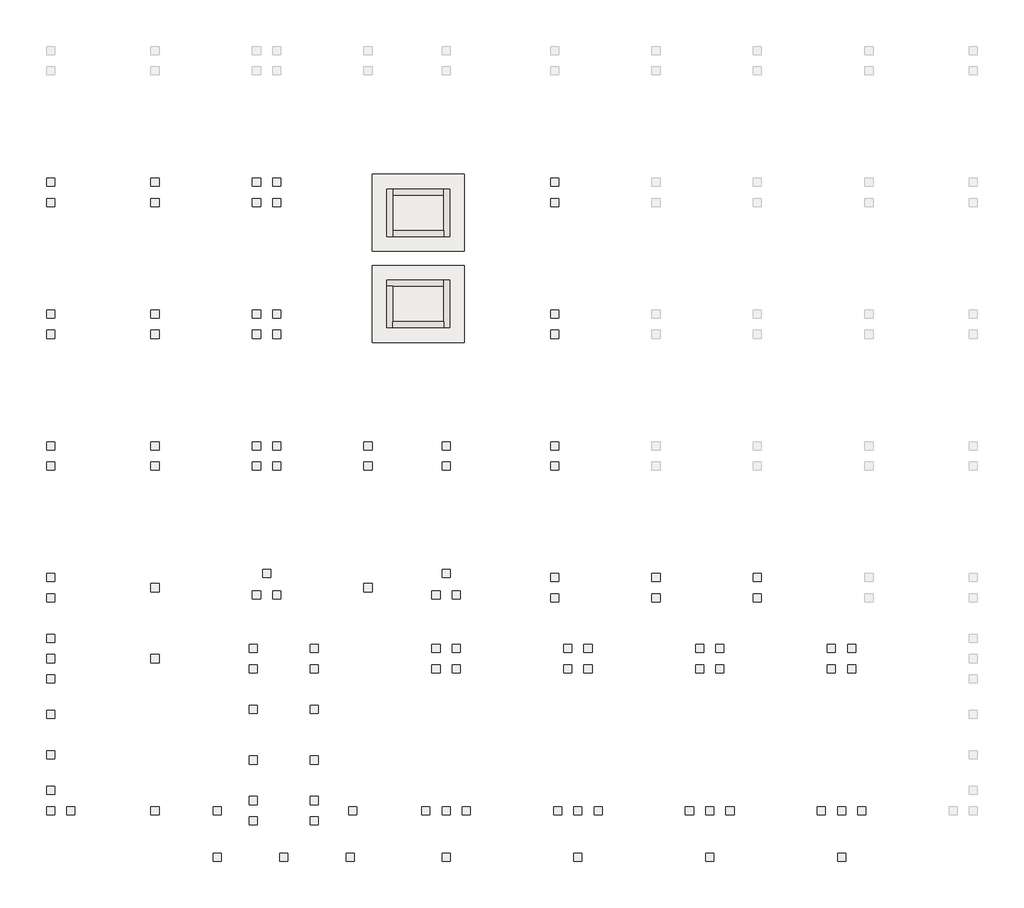
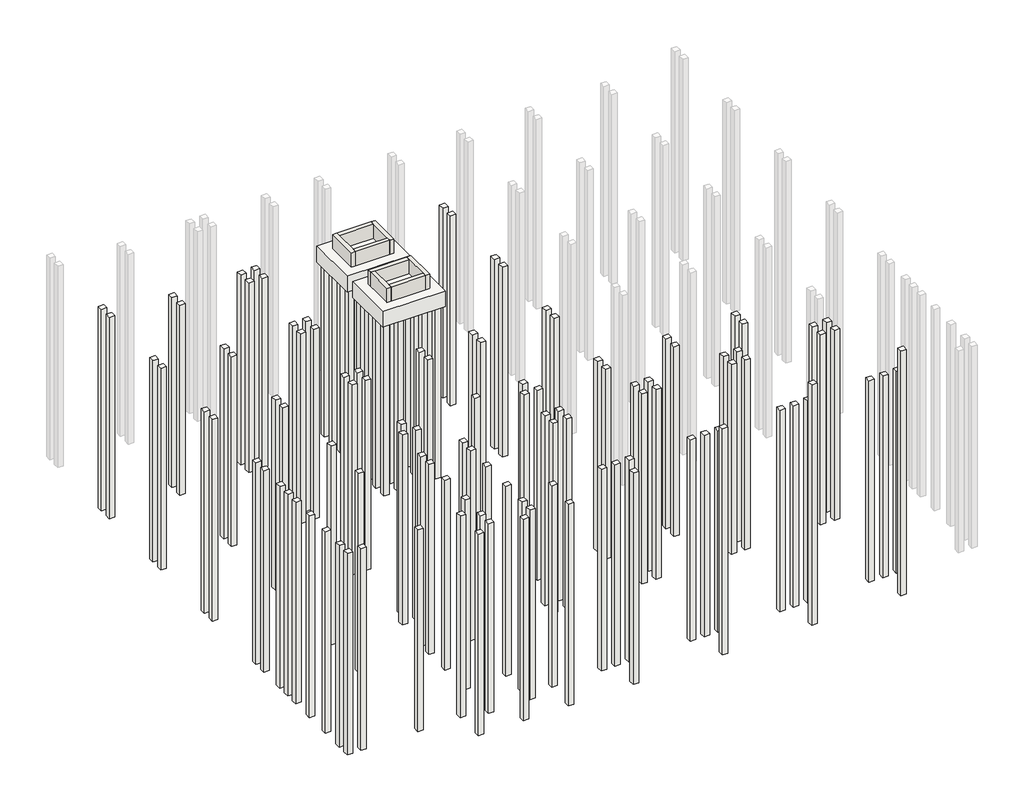
# Not in any storey, part 1 of 2: 143 slabs, 8 walls.
"""IFC4 building model written with IfcOpenShell, lengths in millimetres."""

import ifcopenshell
import ifcopenshell.guid

model = None  # the IFC model being written
_history = None  # IfcOwnerHistory: only IFC2X3 demands one
_inside = {}  # id of a spatial element -> (the spatial element, [elements in it])
_under = {}  # id of a project, library or spatial element -> (it, [spatial elements below it])
_declared = {}  # id of a project -> (the project, [libraries it declares])
_typed = {}  # id of a type object -> (the type object, [elements of that type])
_made_of = {}  # id of a material, layer set ... -> (it, [elements and type objects made of it])


def new_model(schema):
    """Start an empty IFC model of exactly this schema.

    Asked for "IFC4X3", IfcOpenShell would pick the latest addendum, in which some entities
    have other attributes; the version numbers below select the first issue.
    IFC2X3 requires an IfcOwnerHistory on every rooted entity: one is made here for all.
    """
    global model, _history
    if schema == "IFC4X3":
        model = ifcopenshell.file(schema_version=(4, 3, 0, 0))
    else:
        model = ifcopenshell.file(schema=schema)
    _inside.clear()
    _under.clear()
    _declared.clear()
    _typed.clear()
    _made_of.clear()
    _history = None
    if model.schema == "IFC2X3":
        org = make("IfcOrganization", Name="unknown")
        user = make(
            "IfcPersonAndOrganization",
            ThePerson=make("IfcPerson", FamilyName="unknown"),
            TheOrganization=org,
        )
        app = make(
            "IfcApplication",
            ApplicationDeveloper=org,
            Version="unknown",
            ApplicationFullName="unknown",
            ApplicationIdentifier="unknown",
        )
        _history = make(
            "IfcOwnerHistory",
            OwningUser=user,
            OwningApplication=app,
            ChangeAction="ADDED",
            CreationDate=0,
        )
    return model


def make(cls, **values):
    """One entity of the class cls with the attributes given. An attribute that is None is left unset."""
    return model.create_entity(
        cls, **{name: value for name, value in values.items() if value is not None}
    )


def rooted(cls, **values):
    """An entity with a GlobalId (a new one), such as an element, a storey or a relation."""
    return make(cls, GlobalId=ifcopenshell.guid.new(), OwnerHistory=_history, **values)


def si_unit(unit_type, name, prefix=None):
    """IfcSIUnit, for example si_unit("LENGTHUNIT", "METRE", prefix="MILLI")."""
    return make("IfcSIUnit", UnitType=unit_type, Prefix=prefix, Name=name)


def assignment(units):
    """IfcUnitAssignment: the units of a project."""
    return None if units is None else make("IfcUnitAssignment", Units=units)


def point(xyz):
    """IfcCartesianPoint."""
    return None if xyz is None else make("IfcCartesianPoint", Coordinates=xyz)


def direction(xyz):
    """IfcDirection."""
    return None if xyz is None else make("IfcDirection", DirectionRatios=xyz)


def frame(location, z_axis=None, x_axis=None):
    """IfcAxis2Placement3D, a coordinate frame: its origin and axes. An axis left out is left unset."""
    return make(
        "IfcAxis2Placement3D",
        Location=point(location),
        Axis=direction(z_axis),
        RefDirection=direction(x_axis),
    )


def origin():
    """The frame at (0, 0, 0) with its axes left unset."""
    return frame((0.0, 0.0, 0.0))


def place(relative_to, where):
    """IfcLocalPlacement: puts the frame where relative to a parent placement (None: the world)."""
    return make(
        "IfcLocalPlacement", PlacementRelTo=relative_to, RelativePlacement=where
    )


def context(
    kind, dimensions, precision=None, world=None, true_north=None, identifier=None
):
    """IfcGeometricRepresentationContext, for example the 3D "Model" context."""
    return make(
        "IfcGeometricRepresentationContext",
        ContextIdentifier=identifier,
        ContextType=kind,
        CoordinateSpaceDimension=dimensions,
        Precision=precision,
        WorldCoordinateSystem=world,
        TrueNorth=true_north,
    )


def project(units=None, contexts=None):
    """IfcProject with its units and contexts."""
    return rooted(
        "IfcProject",
        Name="project",
        RepresentationContexts=contexts,
        UnitsInContext=assignment(units),
    )


def spatial(cls, under=None, at=None, **own):
    """A site, building, storey or space (cls), placed at a placement, below another one or the project."""
    s = rooted(cls, ObjectPlacement=at, **own)
    if under is not None:
        _under.setdefault(under.id(), (under, []))[1].append(s)
    return s


def polyline(points):
    """IfcPolyline through the points."""
    return make("IfcPolyline", Points=[point(p) for p in points])


def outline(outer, holes=None, kind="AREA"):
    """IfcArbitraryClosedProfileDef: a profile drawn as a closed curve; with holes, ...WithVoids."""
    if holes is None:
        return make("IfcArbitraryClosedProfileDef", ProfileType=kind, OuterCurve=outer)
    return make(
        "IfcArbitraryProfileDefWithVoids",
        ProfileType=kind,
        OuterCurve=outer,
        InnerCurves=holes,
    )


def extrude(swept, where, along, depth):
    """IfcExtrudedAreaSolid: the profile swept, set in the frame where, extruded along a direction by depth."""
    return make(
        "IfcExtrudedAreaSolid",
        SweptArea=swept,
        Position=where,
        ExtrudedDirection=direction(along),
        Depth=depth,
    )


def faces_of(points, faces, orient=None, outer=None):
    """IfcFace entities. A face is a list of loops; a loop is a list of indices into points, from 0.

    orient and outer hold one flag for each loop. By default every Orientation is true, the
    first loop of a face is its IfcFaceOuterBound and the others are IfcFaceBound.
    """
    made = []
    for i, loops in enumerate(faces):
        bounds = []
        for j, loop in enumerate(loops):
            is_outer = j == 0 if outer is None else outer[i][j]
            bounds.append(
                make(
                    "IfcFaceOuterBound" if is_outer else "IfcFaceBound",
                    Bound=make("IfcPolyLoop", Polygon=[points[k] for k in loop]),
                    Orientation=True if orient is None else orient[i][j],
                )
            )
        made.append(make("IfcFace", Bounds=bounds))
    return made


def faceted_brep(points, faces, orient=None, outer=None, voids=None):
    """IfcFacetedBrep: a solid bounded by flat faces; with voids (closed shells), ...WithVoids."""
    shared = [point(p) for p in points]
    hull = make("IfcClosedShell", CfsFaces=faces_of(shared, faces, orient, outer))
    if voids is None:
        return make("IfcFacetedBrep", Outer=hull)
    return make(
        "IfcFacetedBrepWithVoids",
        Outer=hull,
        Voids=[
            make(cls, CfsFaces=faces_of(shared, fs, o, b)) for cls, fs, o, b in voids
        ],
    )


def shape(context_of_items, identifier, shape_type, items):
    """IfcShapeRepresentation: the items that make up one representation, for example the "Body"."""
    return make(
        "IfcShapeRepresentation",
        ContextOfItems=context_of_items,
        RepresentationIdentifier=identifier,
        RepresentationType=shape_type,
        Items=items,
    )


def source(mapping_origin, context_of_items, identifier, shape_type, items):
    """IfcRepresentationMap: a shape defined once, which mapped items show again and again."""
    return make(
        "IfcRepresentationMap",
        MappingOrigin=mapping_origin,
        MappedRepresentation=shape(context_of_items, identifier, shape_type, items),
    )


def transform(
    local_origin,
    x_axis=None,
    y_axis=None,
    z_axis=None,
    scale=None,
    scale2=None,
    scale3=None,
    uniform=True,
):
    """IfcCartesianTransformationOperator3D, or its non-uniform kind. x_axis, y_axis, z_axis: its Axis1, 2, 3."""
    if uniform:
        return make(
            "IfcCartesianTransformationOperator3D",
            Axis1=direction(x_axis),
            Axis2=direction(y_axis),
            LocalOrigin=point(local_origin),
            Scale=scale,
            Axis3=direction(z_axis),
        )
    return make(
        "IfcCartesianTransformationOperator3DnonUniform",
        Axis1=direction(x_axis),
        Axis2=direction(y_axis),
        LocalOrigin=point(local_origin),
        Scale=scale,
        Axis3=direction(z_axis),
        Scale2=scale2,
        Scale3=scale3,
    )


def mapped(mapping_source, mapping_target):
    """IfcMappedItem: shows the shape of a source again, moved by a transform."""
    return make(
        "IfcMappedItem", MappingSource=mapping_source, MappingTarget=mapping_target
    )


def made_of(thing, what):
    """Note that an element or type object is made of a material, layer set ...; save() writes the relation."""
    if what is not None:
        _made_of.setdefault(what.id(), (what, []))[1].append(thing)
    return thing


def element(
    cls,
    number,
    at=None,
    inside=None,
    cuts=None,
    type_object=None,
    material=None,
    context=None,
    identifier="Body",
    shape_type=None,
    held_by="IfcProductDefinitionShape",
    body=None,
    shapes=None,
    **own,
):
    """One element of the class cls, such as IfcWall. Its Tag is "e" and its number.

    at: its placement. inside: the storey or other place that contains it. cuts: it is an
    opening in that element (IfcRelVoidsElement). A single representation is given by context,
    identifier, shape_type and body (its items); several are given by shapes. held_by: the class
    of the entity that holds the representations. save() writes the other relations.
    """
    e = rooted(cls, Tag="e%d" % number, ObjectPlacement=at, **own)
    if body is not None:
        shapes = [shape(context, identifier, shape_type, body)]
    if shapes is not None:
        e.Representation = make(held_by, Representations=shapes)
    if inside is not None:
        _inside.setdefault(inside.id(), (inside, []))[1].append(e)
    if cuts is not None:
        rooted(
            "IfcRelVoidsElement", RelatingBuildingElement=cuts, RelatedOpeningElement=e
        )
    if type_object is not None:
        _typed.setdefault(type_object.id(), (type_object, []))[1].append(e)
    return made_of(e, material)


def aggregate(whole, parts):
    """IfcRelAggregates: a whole, such as a stair, and the parts it consists of."""
    return rooted("IfcRelAggregates", RelatingObject=whole, RelatedObjects=parts)


def save(model, path):
    """Write the relations noted so far, then the file.

    IfcRelAggregates (storeys below a building ...), IfcRelContainedInSpatialStructure (elements
    in a storey), IfcRelDefinesByType, IfcRelAssociatesMaterial and IfcRelDeclares: one each for
    every whole, place, type object, material and project.
    """
    for whole, parts in _under.values():
        aggregate(whole, parts)
    for where, things in _inside.values():
        rooted(
            "IfcRelContainedInSpatialStructure",
            RelatedElements=things,
            RelatingStructure=where,
        )
    for kind, things in _typed.values():
        rooted("IfcRelDefinesByType", RelatedObjects=things, RelatingType=kind)
    for what, things in _made_of.values():
        rooted("IfcRelAssociatesMaterial", RelatedObjects=things, RelatingMaterial=what)
    for by, libraries in _declared.values():
        rooted("IfcRelDeclares", RelatingContext=by, RelatedDefinitions=libraries)
    model.write(path)


def slab_e3f33549(model_context):
    return source(origin(), model_context, "Body", "SweptSolid", [
        extrude(outline(polyline([(200.0, -200.0), (-200.0, -200.0), (-200.0, 200.0), (200.0, 200.0), (200.0, -200.0)])), frame((0.0, 0.0, -20000.0), z_axis=(0.0, 0.0, 1.0), x_axis=(1.0, 0.0, 0.0)), (0.0, 0.0, 1.0), 15320.0),
    ])


def slab_2462c6b3(model_context):
    return source(origin(), model_context, "Body", "SweptSolid", [
        extrude(outline(polyline([(200.0, -200.0), (-200.0, -200.0), (-200.0, 200.0), (200.0, 200.0), (200.0, -200.0)])), frame((0.0, 0.0, -20000.0), z_axis=(0.0, 0.0, 1.0), x_axis=(1.0, 0.0, 0.0)), (0.0, 0.0, 1.0), 14620.0),
    ])


def slab_4eaa82be(model_context):
    return source(origin(), model_context, "Body", "SweptSolid", [
        extrude(outline(polyline([(200.0, -200.0), (-200.0, -200.0), (-200.0, 200.0), (200.0, 200.0), (200.0, -200.0)])), frame((0.0, 0.0, -20000.0), z_axis=(0.0, 0.0, 1.0), x_axis=(1.0, 0.0, 0.0)), (0.0, 0.0, 1.0), 15520.0),
    ])


def slab_98706cf3(model_context):
    return source(origin(), model_context, "Body", "SweptSolid", [
        extrude(outline(polyline([(200.0, -200.0), (-200.0, -200.0), (-200.0, 200.0), (200.0, 200.0), (200.0, -200.0)])), frame((0.0, 0.0, -20000.0), z_axis=(0.0, 0.0, 1.0), x_axis=(1.0, 0.0, 0.0)), (0.0, 0.0, 1.0), 16280.0),
    ])


def slab_73a1868d(model_context):
    return source(origin(), model_context, "Body", "SweptSolid", [
        extrude(outline(polyline([(200.0, -200.0), (-200.0, -200.0), (-200.0, 200.0), (200.0, 200.0), (200.0, -200.0)])), frame((0.0, 0.0, -20000.0), z_axis=(0.0, 0.0, 1.0), x_axis=(1.0, 0.0, 0.0)), (0.0, 0.0, 1.0), 17400.0),
    ])


def slab_81e4ded3(model_context):
    return source(origin(), model_context, "Body", "SweptSolid", [
        extrude(outline(polyline([(200.0, -200.0), (-200.0, -200.0), (-200.0, 200.0), (200.0, 200.0), (200.0, -200.0)])), frame((0.0, 0.0, -20000.0), z_axis=(0.0, 0.0, 1.0), x_axis=(1.0, 0.0, 0.0)), (0.0, 0.0, 1.0), 18520.0),
    ])


def slab_0d914d5e(model_context):
    return source(origin(), model_context, "Body", "SweptSolid", [
        extrude(outline(polyline([(200.0, -200.0), (-200.0, -200.0), (-200.0, 200.0), (200.0, 200.0), (200.0, -200.0)])), frame((0.0, 0.0, -20000.0), z_axis=(0.0, 0.0, 1.0), x_axis=(1.0, 0.0, 0.0)), (0.0, 0.0, 1.0), 18850.0),
    ])


def slab_443494b9(model_context):
    return source(origin(), model_context, "Body", "SweptSolid", [
        extrude(outline(polyline([(200.0, -200.0), (-200.0, -200.0), (-200.0, 200.0), (200.0, 200.0), (200.0, -200.0)])), frame((0.0, 0.0, -20000.0), z_axis=(0.0, 0.0, 1.0), x_axis=(1.0, 0.0, 0.0)), (0.0, 0.0, 1.0), 13220.0),
    ])


model = new_model("IFC4")

# Units and contexts
model_context = context("Model", 3, world=origin())
ifc_project = project(units=[si_unit("LENGTHUNIT", "METRE", prefix="MILLI")], contexts=[model_context])

# Site, building
site = spatial("IfcSite", under=ifc_project)
building = spatial("IfcBuilding", under=site)

# Slabs
placement = place(None, origin())
element("IfcSlab", 1, at=placement, inside=building, context=model_context, shape_type="SweptSolid", body=[
    extrude(outline(polyline([(22350.0, 27600.0), (22350.0, 31400.0), (26900.0, 31400.0), (26900.0, 27600.0), (22350.0, 27600.0)])), frame((0.0, 0.0, -6800.0), z_axis=(0.0, 0.0, 1.0), x_axis=(1.0, 0.0, 0.0)), (0.0, 0.0, 1.0), 1200.0),
])
element("IfcSlab", 2, at=placement, inside=building, context=model_context, shape_type="SweptSolid", body=[
    extrude(outline(polyline([(22350.0, 23100.0), (22350.0, 26900.0), (26900.0, 26900.0), (26900.0, 23100.0), (22350.0, 23100.0)])), frame((0.0, 0.0, -6800.0), z_axis=(0.0, 0.0, 1.0), x_axis=(1.0, 0.0, 0.0)), (0.0, 0.0, 1.0), 1200.0),
])
slab_shape = slab_e3f33549(model_context)
element("IfcSlab", 3, at=placement, inside=building, context=model_context, shape_type="MappedRepresentation", body=[
    mapped(slab_shape, transform((11650.0, 7500.0, 0.0), x_axis=(1.0, 0.0, 0.0), y_axis=(0.0, 1.0, 0.0), z_axis=(0.0, 0.0, 1.0))),
])
element("IfcSlab", 4, at=placement, inside=building, context=model_context, shape_type="MappedRepresentation", body=[
    mapped(slab_shape, transform((11650.0, 11000.0, 0.0), x_axis=(1.0, 0.0, 0.0), y_axis=(0.0, 1.0, 0.0), z_axis=(0.0, 0.0, 1.0))),
])
element("IfcSlab", 5, at=placement, inside=building, context=model_context, shape_type="MappedRepresentation", body=[
    mapped(slab_shape, transform((22150.0, 11000.0, 0.0), x_axis=(1.0, 0.0, 0.0), y_axis=(0.0, 1.0, 0.0), z_axis=(0.0, 0.0, 1.0))),
])
slab_2_shape = slab_2462c6b3(model_context)
element("IfcSlab", 6, at=placement, inside=building, context=model_context, shape_type="MappedRepresentation", body=[
    mapped(slab_2_shape, transform((22150.0, 17000.0, 0.0), x_axis=(1.0, 0.0, 0.0), y_axis=(0.0, 1.0, 0.0), z_axis=(0.0, 0.0, 1.0))),
])
element("IfcSlab", 7, at=placement, inside=building, context=model_context, shape_type="MappedRepresentation", body=[
    mapped(slab_2_shape, transform((22150.0, 18000.0, 0.0), x_axis=(1.0, 0.0, 0.0), y_axis=(0.0, 1.0, 0.0), z_axis=(0.0, 0.0, 1.0))),
])
element("IfcSlab", 8, at=placement, inside=building, context=model_context, shape_type="MappedRepresentation", body=[
    mapped(slab_2_shape, transform((26000.0, 17000.0, 0.0), x_axis=(1.0, 0.0, 0.0), y_axis=(0.0, 1.0, 0.0), z_axis=(0.0, 0.0, 1.0))),
])
element("IfcSlab", 9, at=placement, inside=building, context=model_context, shape_type="MappedRepresentation", body=[
    mapped(slab_2_shape, transform((26000.0, 18000.0, 0.0), x_axis=(1.0, 0.0, 0.0), y_axis=(0.0, 1.0, 0.0), z_axis=(0.0, 0.0, 1.0))),
])
element("IfcSlab", 10, at=placement, inside=building, context=model_context, shape_type="MappedRepresentation", body=[
    mapped(slab_2_shape, transform((11650.0, 17000.0, 0.0), x_axis=(1.0, 0.0, 0.0), y_axis=(0.0, 1.0, 0.0), z_axis=(0.0, 0.0, 1.0))),
])
element("IfcSlab", 11, at=placement, inside=building, context=model_context, shape_type="MappedRepresentation", body=[
    mapped(slab_2_shape, transform((11650.0, 18000.0, 0.0), x_axis=(1.0, 0.0, 0.0), y_axis=(0.0, 1.0, 0.0), z_axis=(0.0, 0.0, 1.0))),
])
element("IfcSlab", 12, at=placement, inside=building, context=model_context, shape_type="MappedRepresentation", body=[
    mapped(slab_2_shape, transform((11650.0, 23500.0, 0.0), x_axis=(1.0, 0.0, 0.0), y_axis=(0.0, 1.0, 0.0), z_axis=(0.0, 0.0, 1.0))),
])
element("IfcSlab", 13, at=placement, inside=building, context=model_context, shape_type="MappedRepresentation", body=[
    mapped(slab_2_shape, transform((11650.0, 24500.0, 0.0), x_axis=(1.0, 0.0, 0.0), y_axis=(0.0, 1.0, 0.0), z_axis=(0.0, 0.0, 1.0))),
])
element("IfcSlab", 14, at=placement, inside=building, context=model_context, shape_type="MappedRepresentation", body=[
    mapped(slab_2_shape, transform((11650.0, 30000.0, 0.0), x_axis=(1.0, 0.0, 0.0), y_axis=(0.0, 1.0, 0.0), z_axis=(0.0, 0.0, 1.0))),
])
element("IfcSlab", 15, at=placement, inside=building, context=model_context, shape_type="MappedRepresentation", body=[
    mapped(slab_2_shape, transform((11650.0, 31000.0, 0.0), x_axis=(1.0, 0.0, 0.0), y_axis=(0.0, 1.0, 0.0), z_axis=(0.0, 0.0, 1.0))),
])
element("IfcSlab", 16, at=placement, inside=building, context=model_context, shape_type="MappedRepresentation", body=[
    mapped(slab_2_shape, transform((31350.0, 10500.0, 0.0), x_axis=(1.0, 0.0, 0.0), y_axis=(0.0, 1.0, 0.0), z_axis=(0.0, 0.0, 1.0))),
])
element("IfcSlab", 17, at=placement, inside=building, context=model_context, shape_type="MappedRepresentation", body=[
    mapped(slab_2_shape, transform((31350.0, 11500.0, 0.0), x_axis=(1.0, 0.0, 0.0), y_axis=(0.0, 1.0, 0.0), z_axis=(0.0, 0.0, 1.0))),
])
element("IfcSlab", 18, at=placement, inside=building, context=model_context, shape_type="MappedRepresentation", body=[
    mapped(slab_2_shape, transform((36350.0, 10500.0, 0.0), x_axis=(1.0, 0.0, 0.0), y_axis=(0.0, 1.0, 0.0), z_axis=(0.0, 0.0, 1.0))),
])
element("IfcSlab", 19, at=placement, inside=building, context=model_context, shape_type="MappedRepresentation", body=[
    mapped(slab_2_shape, transform((36350.0, 11500.0, 0.0), x_axis=(1.0, 0.0, 0.0), y_axis=(0.0, 1.0, 0.0), z_axis=(0.0, 0.0, 1.0))),
])
element("IfcSlab", 20, at=placement, inside=building, context=model_context, shape_type="MappedRepresentation", body=[
    mapped(slab_2_shape, transform((41350.0, 10500.0, 0.0), x_axis=(1.0, 0.0, 0.0), y_axis=(0.0, 1.0, 0.0), z_axis=(0.0, 0.0, 1.0))),
])
element("IfcSlab", 21, at=placement, inside=building, context=model_context, shape_type="MappedRepresentation", body=[
    mapped(slab_2_shape, transform((41350.0, 11500.0, 0.0), x_axis=(1.0, 0.0, 0.0), y_axis=(0.0, 1.0, 0.0), z_axis=(0.0, 0.0, 1.0))),
])
element("IfcSlab", 22, at=placement, inside=building, context=model_context, shape_type="MappedRepresentation", body=[
    mapped(slab_2_shape, transform((46000.0, 7000.0, 0.0), x_axis=(1.0, 0.0, 0.0), y_axis=(0.0, 1.0, 0.0), z_axis=(0.0, 0.0, 1.0))),
])
element("IfcSlab", 23, at=placement, inside=building, context=model_context, shape_type="MappedRepresentation", body=[
    mapped(slab_2_shape, transform((46000.0, 8000.0, 0.0), x_axis=(1.0, 0.0, 0.0), y_axis=(0.0, 1.0, 0.0), z_axis=(0.0, 0.0, 1.0))),
])
element("IfcSlab", 24, at=placement, inside=building, context=model_context, shape_type="MappedRepresentation", body=[
    mapped(slab_2_shape, transform((45000.0, 7000.0, 0.0), x_axis=(1.0, 0.0, 0.0), y_axis=(0.0, 1.0, 0.0), z_axis=(0.0, 0.0, 1.0))),
])
element("IfcSlab", 25, at=placement, inside=building, context=model_context, shape_type="MappedRepresentation", body=[
    mapped(slab_2_shape, transform((45000.0, 8000.0, 0.0), x_axis=(1.0, 0.0, 0.0), y_axis=(0.0, 1.0, 0.0), z_axis=(0.0, 0.0, 1.0))),
])
element("IfcSlab", 26, at=placement, inside=building, context=model_context, shape_type="MappedRepresentation", body=[
    mapped(slab_2_shape, transform((39500.0, 7000.0, 0.0), x_axis=(1.0, 0.0, 0.0), y_axis=(0.0, 1.0, 0.0), z_axis=(0.0, 0.0, 1.0))),
])
element("IfcSlab", 27, at=placement, inside=building, context=model_context, shape_type="MappedRepresentation", body=[
    mapped(slab_2_shape, transform((39500.0, 8000.0, 0.0), x_axis=(1.0, 0.0, 0.0), y_axis=(0.0, 1.0, 0.0), z_axis=(0.0, 0.0, 1.0))),
])
element("IfcSlab", 28, at=placement, inside=building, context=model_context, shape_type="MappedRepresentation", body=[
    mapped(slab_2_shape, transform((38500.0, 7000.0, 0.0), x_axis=(1.0, 0.0, 0.0), y_axis=(0.0, 1.0, 0.0), z_axis=(0.0, 0.0, 1.0))),
])
element("IfcSlab", 29, at=placement, inside=building, context=model_context, shape_type="MappedRepresentation", body=[
    mapped(slab_2_shape, transform((38500.0, 8000.0, 0.0), x_axis=(1.0, 0.0, 0.0), y_axis=(0.0, 1.0, 0.0), z_axis=(0.0, 0.0, 1.0))),
])
element("IfcSlab", 30, at=placement, inside=building, context=model_context, shape_type="MappedRepresentation", body=[
    mapped(slab_2_shape, transform((33000.0, 7000.0, 0.0), x_axis=(1.0, 0.0, 0.0), y_axis=(0.0, 1.0, 0.0), z_axis=(0.0, 0.0, 1.0))),
])
element("IfcSlab", 31, at=placement, inside=building, context=model_context, shape_type="MappedRepresentation", body=[
    mapped(slab_2_shape, transform((33000.0, 8000.0, 0.0), x_axis=(1.0, 0.0, 0.0), y_axis=(0.0, 1.0, 0.0), z_axis=(0.0, 0.0, 1.0))),
])
element("IfcSlab", 32, at=placement, inside=building, context=model_context, shape_type="MappedRepresentation", body=[
    mapped(slab_2_shape, transform((32000.0, 7000.0, 0.0), x_axis=(1.0, 0.0, 0.0), y_axis=(0.0, 1.0, 0.0), z_axis=(0.0, 0.0, 1.0))),
])
element("IfcSlab", 33, at=placement, inside=building, context=model_context, shape_type="MappedRepresentation", body=[
    mapped(slab_2_shape, transform((32000.0, 8000.0, 0.0), x_axis=(1.0, 0.0, 0.0), y_axis=(0.0, 1.0, 0.0), z_axis=(0.0, 0.0, 1.0))),
])
element("IfcSlab", 34, at=placement, inside=building, context=model_context, shape_type="MappedRepresentation", body=[
    mapped(slab_2_shape, transform((26500.0, 7000.0, 0.0), x_axis=(1.0, 0.0, 0.0), y_axis=(0.0, 1.0, 0.0), z_axis=(0.0, 0.0, 1.0))),
])
element("IfcSlab", 35, at=placement, inside=building, context=model_context, shape_type="MappedRepresentation", body=[
    mapped(slab_2_shape, transform((26500.0, 8000.0, 0.0), x_axis=(1.0, 0.0, 0.0), y_axis=(0.0, 1.0, 0.0), z_axis=(0.0, 0.0, 1.0))),
])
element("IfcSlab", 36, at=placement, inside=building, context=model_context, shape_type="MappedRepresentation", body=[
    mapped(slab_2_shape, transform((25500.0, 7000.0, 0.0), x_axis=(1.0, 0.0, 0.0), y_axis=(0.0, 1.0, 0.0), z_axis=(0.0, 0.0, 1.0))),
])
element("IfcSlab", 37, at=placement, inside=building, context=model_context, shape_type="MappedRepresentation", body=[
    mapped(slab_2_shape, transform((25500.0, 8000.0, 0.0), x_axis=(1.0, 0.0, 0.0), y_axis=(0.0, 1.0, 0.0), z_axis=(0.0, 0.0, 1.0))),
])
element("IfcSlab", 38, at=placement, inside=building, context=model_context, shape_type="MappedRepresentation", body=[
    mapped(slab_2_shape, transform((17650.0, 30000.0, 0.0), x_axis=(1.0, 0.0, 0.0), y_axis=(0.0, 1.0, 0.0), z_axis=(0.0, 0.0, 1.0))),
])
element("IfcSlab", 39, at=placement, inside=building, context=model_context, shape_type="MappedRepresentation", body=[
    mapped(slab_2_shape, transform((17650.0, 31000.0, 0.0), x_axis=(1.0, 0.0, 0.0), y_axis=(0.0, 1.0, 0.0), z_axis=(0.0, 0.0, 1.0))),
])
element("IfcSlab", 40, at=placement, inside=building, context=model_context, shape_type="MappedRepresentation", body=[
    mapped(slab_2_shape, transform((16650.0, 30000.0, 0.0), x_axis=(1.0, 0.0, 0.0), y_axis=(0.0, 1.0, 0.0), z_axis=(0.0, 0.0, 1.0))),
])
element("IfcSlab", 41, at=placement, inside=building, context=model_context, shape_type="MappedRepresentation", body=[
    mapped(slab_2_shape, transform((16650.0, 31000.0, 0.0), x_axis=(1.0, 0.0, 0.0), y_axis=(0.0, 1.0, 0.0), z_axis=(0.0, 0.0, 1.0))),
])
element("IfcSlab", 42, at=placement, inside=building, context=model_context, shape_type="MappedRepresentation", body=[
    mapped(slab_2_shape, transform((17650.0, 23500.0, 0.0), x_axis=(1.0, 0.0, 0.0), y_axis=(0.0, 1.0, 0.0), z_axis=(0.0, 0.0, 1.0))),
])
element("IfcSlab", 43, at=placement, inside=building, context=model_context, shape_type="MappedRepresentation", body=[
    mapped(slab_2_shape, transform((17650.0, 24500.0, 0.0), x_axis=(1.0, 0.0, 0.0), y_axis=(0.0, 1.0, 0.0), z_axis=(0.0, 0.0, 1.0))),
])
element("IfcSlab", 44, at=placement, inside=building, context=model_context, shape_type="MappedRepresentation", body=[
    mapped(slab_2_shape, transform((16650.0, 23500.0, 0.0), x_axis=(1.0, 0.0, 0.0), y_axis=(0.0, 1.0, 0.0), z_axis=(0.0, 0.0, 1.0))),
])
element("IfcSlab", 45, at=placement, inside=building, context=model_context, shape_type="MappedRepresentation", body=[
    mapped(slab_2_shape, transform((16650.0, 24500.0, 0.0), x_axis=(1.0, 0.0, 0.0), y_axis=(0.0, 1.0, 0.0), z_axis=(0.0, 0.0, 1.0))),
])
element("IfcSlab", 46, at=placement, inside=building, context=model_context, shape_type="MappedRepresentation", body=[
    mapped(slab_2_shape, transform((17650.0, 17000.0, 0.0), x_axis=(1.0, 0.0, 0.0), y_axis=(0.0, 1.0, 0.0), z_axis=(0.0, 0.0, 1.0))),
])
element("IfcSlab", 47, at=placement, inside=building, context=model_context, shape_type="MappedRepresentation", body=[
    mapped(slab_2_shape, transform((17650.0, 18000.0, 0.0), x_axis=(1.0, 0.0, 0.0), y_axis=(0.0, 1.0, 0.0), z_axis=(0.0, 0.0, 1.0))),
])
element("IfcSlab", 48, at=placement, inside=building, context=model_context, shape_type="MappedRepresentation", body=[
    mapped(slab_2_shape, transform((16650.0, 17000.0, 0.0), x_axis=(1.0, 0.0, 0.0), y_axis=(0.0, 1.0, 0.0), z_axis=(0.0, 0.0, 1.0))),
])
element("IfcSlab", 49, at=placement, inside=building, context=model_context, shape_type="MappedRepresentation", body=[
    mapped(slab_2_shape, transform((16650.0, 18000.0, 0.0), x_axis=(1.0, 0.0, 0.0), y_axis=(0.0, 1.0, 0.0), z_axis=(0.0, 0.0, 1.0))),
])
element("IfcSlab", 50, at=placement, inside=building, context=model_context, shape_type="MappedRepresentation", body=[
    mapped(slab_2_shape, transform((16650.0, 10650.0, 0.0), x_axis=(1.0, 0.0, 0.0), y_axis=(0.0, 1.0, 0.0), z_axis=(0.0, 0.0, 1.0))),
])
element("IfcSlab", 51, at=placement, inside=building, context=model_context, shape_type="MappedRepresentation", body=[
    mapped(slab_2_shape, transform((17650.0, 10650.0, 0.0), x_axis=(1.0, 0.0, 0.0), y_axis=(0.0, 1.0, 0.0), z_axis=(0.0, 0.0, 1.0))),
])
element("IfcSlab", 52, at=placement, inside=building, context=model_context, shape_type="MappedRepresentation", body=[
    mapped(slab_2_shape, transform((17150.0, 11700.0, 0.0), x_axis=(1.0, 0.0, 0.0), y_axis=(0.0, 1.0, 0.0), z_axis=(0.0, 0.0, 1.0))),
])
element("IfcSlab", 53, at=placement, inside=building, context=model_context, shape_type="MappedRepresentation", body=[
    mapped(slab_2_shape, transform((19500.0, 7000.0, 0.0), x_axis=(1.0, 0.0, 0.0), y_axis=(0.0, 1.0, 0.0), z_axis=(0.0, 0.0, 1.0))),
])
element("IfcSlab", 54, at=placement, inside=building, context=model_context, shape_type="MappedRepresentation", body=[
    mapped(slab_2_shape, transform((19500.0, 8000.0, 0.0), x_axis=(1.0, 0.0, 0.0), y_axis=(0.0, 1.0, 0.0), z_axis=(0.0, 0.0, 1.0))),
])
element("IfcSlab", 55, at=placement, inside=building, context=model_context, shape_type="MappedRepresentation", body=[
    mapped(slab_2_shape, transform((16500.0, 7000.0, 0.0), x_axis=(1.0, 0.0, 0.0), y_axis=(0.0, 1.0, 0.0), z_axis=(0.0, 0.0, 1.0))),
])
element("IfcSlab", 56, at=placement, inside=building, context=model_context, shape_type="MappedRepresentation", body=[
    mapped(slab_2_shape, transform((16500.0, 8000.0, 0.0), x_axis=(1.0, 0.0, 0.0), y_axis=(0.0, 1.0, 0.0), z_axis=(0.0, 0.0, 1.0))),
])
element("IfcSlab", 57, at=placement, inside=building, context=model_context, shape_type="MappedRepresentation", body=[
    mapped(slab_2_shape, transform((19500.0, -500.0, 0.0), x_axis=(1.0, 0.0, 0.0), y_axis=(0.0, 1.0, 0.0), z_axis=(0.0, 0.0, 1.0))),
])
element("IfcSlab", 58, at=placement, inside=building, context=model_context, shape_type="MappedRepresentation", body=[
    mapped(slab_2_shape, transform((19500.0, 500.0, 0.0), x_axis=(1.0, 0.0, 0.0), y_axis=(0.0, 1.0, 0.0), z_axis=(0.0, 0.0, 1.0))),
])
element("IfcSlab", 59, at=placement, inside=building, context=model_context, shape_type="MappedRepresentation", body=[
    mapped(slab_2_shape, transform((16500.0, -500.0, 0.0), x_axis=(1.0, 0.0, 0.0), y_axis=(0.0, 1.0, 0.0), z_axis=(0.0, 0.0, 1.0))),
])
element("IfcSlab", 60, at=placement, inside=building, context=model_context, shape_type="MappedRepresentation", body=[
    mapped(slab_2_shape, transform((16500.0, 500.0, 0.0), x_axis=(1.0, 0.0, 0.0), y_axis=(0.0, 1.0, 0.0), z_axis=(0.0, 0.0, 1.0))),
])
element("IfcSlab", 61, at=placement, inside=building, context=model_context, shape_type="MappedRepresentation", body=[
    mapped(slab_2_shape, transform((16500.0, 5000.0, 0.0), x_axis=(1.0, 0.0, 0.0), y_axis=(0.0, 1.0, 0.0), z_axis=(0.0, 0.0, 1.0))),
])
element("IfcSlab", 62, at=placement, inside=building, context=model_context, shape_type="MappedRepresentation", body=[
    mapped(slab_2_shape, transform((19500.0, 5000.0, 0.0), x_axis=(1.0, 0.0, 0.0), y_axis=(0.0, 1.0, 0.0), z_axis=(0.0, 0.0, 1.0))),
])
element("IfcSlab", 63, at=placement, inside=building, context=model_context, shape_type="MappedRepresentation", body=[
    mapped(slab_2_shape, transform((19500.0, 2500.0, 0.0), x_axis=(1.0, 0.0, 0.0), y_axis=(0.0, 1.0, 0.0), z_axis=(0.0, 0.0, 1.0))),
])
element("IfcSlab", 64, at=placement, inside=building, context=model_context, shape_type="MappedRepresentation", body=[
    mapped(slab_2_shape, transform((16500.0, 2500.0, 0.0), x_axis=(1.0, 0.0, 0.0), y_axis=(0.0, 1.0, 0.0), z_axis=(0.0, 0.0, 1.0))),
])
element("IfcSlab", 65, at=placement, inside=building, context=model_context, shape_type="MappedRepresentation", body=[
    mapped(slab_2_shape, transform((25500.0, 10650.0, 0.0), x_axis=(1.0, 0.0, 0.0), y_axis=(0.0, 1.0, 0.0), z_axis=(0.0, 0.0, 1.0))),
])
element("IfcSlab", 66, at=placement, inside=building, context=model_context, shape_type="MappedRepresentation", body=[
    mapped(slab_2_shape, transform((26500.0, 10650.0, 0.0), x_axis=(1.0, 0.0, 0.0), y_axis=(0.0, 1.0, 0.0), z_axis=(0.0, 0.0, 1.0))),
])
element("IfcSlab", 67, at=placement, inside=building, context=model_context, shape_type="MappedRepresentation", body=[
    mapped(slab_2_shape, transform((26000.0, 11700.0, 0.0), x_axis=(1.0, 0.0, 0.0), y_axis=(0.0, 1.0, 0.0), z_axis=(0.0, 0.0, 1.0))),
])
element("IfcSlab", 68, at=placement, inside=building, context=model_context, shape_type="MappedRepresentation", body=[
    mapped(slab_2_shape, transform((31350.0, 17000.0, 0.0), x_axis=(1.0, 0.0, 0.0), y_axis=(0.0, 1.0, 0.0), z_axis=(0.0, 0.0, 1.0))),
])
element("IfcSlab", 69, at=placement, inside=building, context=model_context, shape_type="MappedRepresentation", body=[
    mapped(slab_2_shape, transform((31350.0, 18000.0, 0.0), x_axis=(1.0, 0.0, 0.0), y_axis=(0.0, 1.0, 0.0), z_axis=(0.0, 0.0, 1.0))),
])
element("IfcSlab", 70, at=placement, inside=building, context=model_context, shape_type="MappedRepresentation", body=[
    mapped(slab_2_shape, transform((31350.0, 23500.0, 0.0), x_axis=(1.0, 0.0, 0.0), y_axis=(0.0, 1.0, 0.0), z_axis=(0.0, 0.0, 1.0))),
])
element("IfcSlab", 71, at=placement, inside=building, context=model_context, shape_type="MappedRepresentation", body=[
    mapped(slab_2_shape, transform((31350.0, 24500.0, 0.0), x_axis=(1.0, 0.0, 0.0), y_axis=(0.0, 1.0, 0.0), z_axis=(0.0, 0.0, 1.0))),
])
element("IfcSlab", 72, at=placement, inside=building, context=model_context, shape_type="MappedRepresentation", body=[
    mapped(slab_2_shape, transform((31350.0, 30000.0, 0.0), x_axis=(1.0, 0.0, 0.0), y_axis=(0.0, 1.0, 0.0), z_axis=(0.0, 0.0, 1.0))),
])
element("IfcSlab", 73, at=placement, inside=building, context=model_context, shape_type="MappedRepresentation", body=[
    mapped(slab_2_shape, transform((31350.0, 31000.0, 0.0), x_axis=(1.0, 0.0, 0.0), y_axis=(0.0, 1.0, 0.0), z_axis=(0.0, 0.0, 1.0))),
])
slab_3_shape = slab_4eaa82be(model_context)
element("IfcSlab", 74, at=placement, inside=building, context=model_context, shape_type="MappedRepresentation", body=[
    mapped(slab_3_shape, transform((6500.0, 8500.0, 0.0), x_axis=(1.0, 0.0, 0.0), y_axis=(0.0, 1.0, 0.0), z_axis=(0.0, 0.0, 1.0))),
])
element("IfcSlab", 75, at=placement, inside=building, context=model_context, shape_type="MappedRepresentation", body=[
    mapped(slab_3_shape, transform((6500.0, 7500.0, 0.0), x_axis=(1.0, 0.0, 0.0), y_axis=(0.0, 1.0, 0.0), z_axis=(0.0, 0.0, 1.0))),
])
element("IfcSlab", 76, at=placement, inside=building, context=model_context, shape_type="MappedRepresentation", body=[
    mapped(slab_3_shape, transform((6500.0, 6500.0, 0.0), x_axis=(1.0, 0.0, 0.0), y_axis=(0.0, 1.0, 0.0), z_axis=(0.0, 0.0, 1.0))),
])
element("IfcSlab", 77, at=placement, inside=building, context=model_context, shape_type="MappedRepresentation", body=[
    mapped(slab_3_shape, transform((6500.0, 0.0, 0.0), x_axis=(1.0, 0.0, 0.0), y_axis=(0.0, 1.0, 0.0), z_axis=(0.0, 0.0, 1.0))),
])
element("IfcSlab", 78, at=placement, inside=building, context=model_context, shape_type="MappedRepresentation", body=[
    mapped(slab_3_shape, transform((6500.0, 1000.0, 0.0), x_axis=(1.0, 0.0, 0.0), y_axis=(0.0, 1.0, 0.0), z_axis=(0.0, 0.0, 1.0))),
])
element("IfcSlab", 79, at=placement, inside=building, context=model_context, shape_type="MappedRepresentation", body=[
    mapped(slab_3_shape, transform((7500.0, 0.0, 0.0), x_axis=(1.0, 0.0, 0.0), y_axis=(0.0, 1.0, 0.0), z_axis=(0.0, 0.0, 1.0))),
])
element("IfcSlab", 80, at=placement, inside=building, context=model_context, shape_type="MappedRepresentation", body=[
    mapped(slab_3_shape, transform((6500.0, 4750.0, 0.0), x_axis=(1.0, 0.0, 0.0), y_axis=(0.0, 1.0, 0.0), z_axis=(0.0, 0.0, 1.0))),
])
element("IfcSlab", 81, at=placement, inside=building, context=model_context, shape_type="MappedRepresentation", body=[
    mapped(slab_3_shape, transform((6500.0, 2750.0, 0.0), x_axis=(1.0, 0.0, 0.0), y_axis=(0.0, 1.0, 0.0), z_axis=(0.0, 0.0, 1.0))),
])
element("IfcSlab", 82, at=placement, inside=building, context=model_context, shape_type="MappedRepresentation", body=[
    mapped(slab_3_shape, transform((14725.0, 0.0, 0.0), x_axis=(1.0, 0.0, 0.0), y_axis=(0.0, 1.0, 0.0), z_axis=(0.0, 0.0, 1.0))),
])
element("IfcSlab", 83, at=placement, inside=building, context=model_context, shape_type="MappedRepresentation", body=[
    mapped(slab_3_shape, transform((11650.0, 0.0, 0.0), x_axis=(1.0, 0.0, 0.0), y_axis=(0.0, 1.0, 0.0), z_axis=(0.0, 0.0, 1.0))),
])
element("IfcSlab", 84, at=placement, inside=building, context=model_context, shape_type="MappedRepresentation", body=[
    mapped(slab_3_shape, transform((45500.0, 0.0, 0.0), x_axis=(1.0, 0.0, 0.0), y_axis=(0.0, 1.0, 0.0), z_axis=(0.0, 0.0, 1.0))),
])
element("IfcSlab", 85, at=placement, inside=building, context=model_context, shape_type="MappedRepresentation", body=[
    mapped(slab_3_shape, transform((46500.0, 0.0, 0.0), x_axis=(1.0, 0.0, 0.0), y_axis=(0.0, 1.0, 0.0), z_axis=(0.0, 0.0, 1.0))),
])
element("IfcSlab", 86, at=placement, inside=building, context=model_context, shape_type="MappedRepresentation", body=[
    mapped(slab_3_shape, transform((44500.0, 0.0, 0.0), x_axis=(1.0, 0.0, 0.0), y_axis=(0.0, 1.0, 0.0), z_axis=(0.0, 0.0, 1.0))),
])
element("IfcSlab", 87, at=placement, inside=building, context=model_context, shape_type="MappedRepresentation", body=[
    mapped(slab_3_shape, transform((39000.0, 0.0, 0.0), x_axis=(1.0, 0.0, 0.0), y_axis=(0.0, 1.0, 0.0), z_axis=(0.0, 0.0, 1.0))),
])
element("IfcSlab", 88, at=placement, inside=building, context=model_context, shape_type="MappedRepresentation", body=[
    mapped(slab_3_shape, transform((40000.0, 0.0, 0.0), x_axis=(1.0, 0.0, 0.0), y_axis=(0.0, 1.0, 0.0), z_axis=(0.0, 0.0, 1.0))),
])
element("IfcSlab", 89, at=placement, inside=building, context=model_context, shape_type="MappedRepresentation", body=[
    mapped(slab_3_shape, transform((38000.0, 0.0, 0.0), x_axis=(1.0, 0.0, 0.0), y_axis=(0.0, 1.0, 0.0), z_axis=(0.0, 0.0, 1.0))),
])
element("IfcSlab", 90, at=placement, inside=building, context=model_context, shape_type="MappedRepresentation", body=[
    mapped(slab_3_shape, transform((32500.0, 0.0, 0.0), x_axis=(1.0, 0.0, 0.0), y_axis=(0.0, 1.0, 0.0), z_axis=(0.0, 0.0, 1.0))),
])
element("IfcSlab", 91, at=placement, inside=building, context=model_context, shape_type="MappedRepresentation", body=[
    mapped(slab_3_shape, transform((33500.0, 0.0, 0.0), x_axis=(1.0, 0.0, 0.0), y_axis=(0.0, 1.0, 0.0), z_axis=(0.0, 0.0, 1.0))),
])
element("IfcSlab", 92, at=placement, inside=building, context=model_context, shape_type="MappedRepresentation", body=[
    mapped(slab_3_shape, transform((31500.0, 0.0, 0.0), x_axis=(1.0, 0.0, 0.0), y_axis=(0.0, 1.0, 0.0), z_axis=(0.0, 0.0, 1.0))),
])
element("IfcSlab", 93, at=placement, inside=building, context=model_context, shape_type="MappedRepresentation", body=[
    mapped(slab_3_shape, transform((26000.0, 0.0, 0.0), x_axis=(1.0, 0.0, 0.0), y_axis=(0.0, 1.0, 0.0), z_axis=(0.0, 0.0, 1.0))),
])
element("IfcSlab", 94, at=placement, inside=building, context=model_context, shape_type="MappedRepresentation", body=[
    mapped(slab_3_shape, transform((27000.0, 0.0, 0.0), x_axis=(1.0, 0.0, 0.0), y_axis=(0.0, 1.0, 0.0), z_axis=(0.0, 0.0, 1.0))),
])
element("IfcSlab", 95, at=placement, inside=building, context=model_context, shape_type="MappedRepresentation", body=[
    mapped(slab_3_shape, transform((25000.0, 0.0, 0.0), x_axis=(1.0, 0.0, 0.0), y_axis=(0.0, 1.0, 0.0), z_axis=(0.0, 0.0, 1.0))),
])
element("IfcSlab", 96, at=placement, inside=building, context=model_context, shape_type="MappedRepresentation", body=[
    mapped(slab_3_shape, transform((21400.0, 0.0, 0.0), x_axis=(1.0, 0.0, 0.0), y_axis=(0.0, 1.0, 0.0), z_axis=(0.0, 0.0, 1.0))),
])
element("IfcSlab", 97, at=placement, inside=building, context=model_context, shape_type="MappedRepresentation", body=[
    mapped(slab_3_shape, transform((6500.0, 10500.0, 0.0), x_axis=(1.0, 0.0, 0.0), y_axis=(0.0, 1.0, 0.0), z_axis=(0.0, 0.0, 1.0))),
])
element("IfcSlab", 98, at=placement, inside=building, context=model_context, shape_type="MappedRepresentation", body=[
    mapped(slab_3_shape, transform((6500.0, 11500.0, 0.0), x_axis=(1.0, 0.0, 0.0), y_axis=(0.0, 1.0, 0.0), z_axis=(0.0, 0.0, 1.0))),
])
element("IfcSlab", 99, at=placement, inside=building, context=model_context, shape_type="MappedRepresentation", body=[
    mapped(slab_3_shape, transform((6500.0, 17000.0, 0.0), x_axis=(1.0, 0.0, 0.0), y_axis=(0.0, 1.0, 0.0), z_axis=(0.0, 0.0, 1.0))),
])
element("IfcSlab", 100, at=placement, inside=building, context=model_context, shape_type="MappedRepresentation", body=[
    mapped(slab_3_shape, transform((6500.0, 18000.0, 0.0), x_axis=(1.0, 0.0, 0.0), y_axis=(0.0, 1.0, 0.0), z_axis=(0.0, 0.0, 1.0))),
])
element("IfcSlab", 101, at=placement, inside=building, context=model_context, shape_type="MappedRepresentation", body=[
    mapped(slab_3_shape, transform((6500.0, 23500.0, 0.0), x_axis=(1.0, 0.0, 0.0), y_axis=(0.0, 1.0, 0.0), z_axis=(0.0, 0.0, 1.0))),
])
element("IfcSlab", 102, at=placement, inside=building, context=model_context, shape_type="MappedRepresentation", body=[
    mapped(slab_3_shape, transform((6500.0, 24500.0, 0.0), x_axis=(1.0, 0.0, 0.0), y_axis=(0.0, 1.0, 0.0), z_axis=(0.0, 0.0, 1.0))),
])
element("IfcSlab", 103, at=placement, inside=building, context=model_context, shape_type="MappedRepresentation", body=[
    mapped(slab_3_shape, transform((6500.0, 30000.0, 0.0), x_axis=(1.0, 0.0, 0.0), y_axis=(0.0, 1.0, 0.0), z_axis=(0.0, 0.0, 1.0))),
])
element("IfcSlab", 104, at=placement, inside=building, context=model_context, shape_type="MappedRepresentation", body=[
    mapped(slab_3_shape, transform((6500.0, 31000.0, 0.0), x_axis=(1.0, 0.0, 0.0), y_axis=(0.0, 1.0, 0.0), z_axis=(0.0, 0.0, 1.0))),
])
element("IfcSlab", 105, at=placement, inside=building, context=model_context, shape_type="MappedRepresentation", body=[
    mapped(slab_3_shape, transform((14725.0, -2300.0, 0.0), x_axis=(1.0, 0.0, 0.0), y_axis=(0.0, 1.0, 0.0), z_axis=(0.0, 0.0, 1.0))),
])
element("IfcSlab", 106, at=placement, inside=building, context=model_context, shape_type="MappedRepresentation", body=[
    mapped(slab_3_shape, transform((21275.0, -2300.0, 0.0), x_axis=(1.0, 0.0, 0.0), y_axis=(0.0, 1.0, 0.0), z_axis=(0.0, 0.0, 1.0))),
])
element("IfcSlab", 107, at=placement, inside=building, context=model_context, shape_type="MappedRepresentation", body=[
    mapped(slab_3_shape, transform((18000.0, -2300.0, 0.0), x_axis=(1.0, 0.0, 0.0), y_axis=(0.0, 1.0, 0.0), z_axis=(0.0, 0.0, 1.0))),
])
slab_4_shape = slab_98706cf3(model_context)
element("IfcSlab", 108, at=placement, inside=building, context=model_context, shape_type="MappedRepresentation", body=[
    mapped(slab_4_shape, transform((26000.0, -2300.0, 0.0), x_axis=(1.0, 0.0, 0.0), y_axis=(0.0, 1.0, 0.0), z_axis=(0.0, 0.0, 1.0))),
])
slab_5_shape = slab_73a1868d(model_context)
element("IfcSlab", 109, at=placement, inside=building, context=model_context, shape_type="MappedRepresentation", body=[
    mapped(slab_5_shape, transform((32500.0, -2300.0, 0.0), x_axis=(1.0, 0.0, 0.0), y_axis=(0.0, 1.0, 0.0), z_axis=(0.0, 0.0, 1.0))),
])
slab_6_shape = slab_81e4ded3(model_context)
element("IfcSlab", 110, at=placement, inside=building, context=model_context, shape_type="MappedRepresentation", body=[
    mapped(slab_6_shape, transform((39000.0, -2300.0, 0.0), x_axis=(1.0, 0.0, 0.0), y_axis=(0.0, 1.0, 0.0), z_axis=(0.0, 0.0, 1.0))),
])
slab_7_shape = slab_0d914d5e(model_context)
element("IfcSlab", 111, at=placement, inside=building, context=model_context, shape_type="MappedRepresentation", body=[
    mapped(slab_7_shape, transform((45500.0, -2300.0, 0.0), x_axis=(1.0, 0.0, 0.0), y_axis=(0.0, 1.0, 0.0), z_axis=(0.0, 0.0, 1.0))),
])
slab_8_shape = slab_443494b9(model_context)
element("IfcSlab", 112, at=placement, inside=building, context=model_context, shape_type="MappedRepresentation", body=[
    mapped(slab_8_shape, transform((23750.0, 31000.0, 0.0), x_axis=(1.0, 0.0, 0.0), y_axis=(0.0, 1.0, 0.0), z_axis=(0.0, 0.0, 1.0))),
])
element("IfcSlab", 113, at=placement, inside=building, context=model_context, shape_type="MappedRepresentation", body=[
    mapped(slab_8_shape, transform((23750.0, 29000.0, 0.0), x_axis=(1.0, 0.0, 0.0), y_axis=(0.0, 1.0, 0.0), z_axis=(0.0, 0.0, 1.0))),
])
element("IfcSlab", 114, at=placement, inside=building, context=model_context, shape_type="MappedRepresentation", body=[
    mapped(slab_8_shape, transform((22750.0, 29000.0, 0.0), x_axis=(1.0, 0.0, 0.0), y_axis=(0.0, 1.0, 0.0), z_axis=(0.0, 0.0, 1.0))),
])
element("IfcSlab", 115, at=placement, inside=building, context=model_context, shape_type="MappedRepresentation", body=[
    mapped(slab_8_shape, transform((22750.0, 31000.0, 0.0), x_axis=(1.0, 0.0, 0.0), y_axis=(0.0, 1.0, 0.0), z_axis=(0.0, 0.0, 1.0))),
])
element("IfcSlab", 116, at=placement, inside=building, context=model_context, shape_type="MappedRepresentation", body=[
    mapped(slab_8_shape, transform((23750.0, 30000.0, 0.0), x_axis=(1.0, 0.0, 0.0), y_axis=(0.0, 1.0, 0.0), z_axis=(0.0, 0.0, 1.0))),
])
element("IfcSlab", 117, at=placement, inside=building, context=model_context, shape_type="MappedRepresentation", body=[
    mapped(slab_8_shape, transform((22750.0, 30000.0, 0.0), x_axis=(1.0, 0.0, 0.0), y_axis=(0.0, 1.0, 0.0), z_axis=(0.0, 0.0, 1.0))),
])
element("IfcSlab", 118, at=placement, inside=building, context=model_context, shape_type="MappedRepresentation", body=[
    mapped(slab_8_shape, transform((23750.0, 28000.0, 0.0), x_axis=(1.0, 0.0, 0.0), y_axis=(0.0, 1.0, 0.0), z_axis=(0.0, 0.0, 1.0))),
])
element("IfcSlab", 119, at=placement, inside=building, context=model_context, shape_type="MappedRepresentation", body=[
    mapped(slab_8_shape, transform((22750.0, 28000.0, 0.0), x_axis=(1.0, 0.0, 0.0), y_axis=(0.0, 1.0, 0.0), z_axis=(0.0, 0.0, 1.0))),
])
element("IfcSlab", 120, at=placement, inside=building, context=model_context, shape_type="MappedRepresentation", body=[
    mapped(slab_8_shape, transform((26500.0, 31000.0, 0.0), x_axis=(1.0, 0.0, 0.0), y_axis=(0.0, 1.0, 0.0), z_axis=(0.0, 0.0, 1.0))),
])
element("IfcSlab", 121, at=placement, inside=building, context=model_context, shape_type="MappedRepresentation", body=[
    mapped(slab_8_shape, transform((26500.0, 29000.0, 0.0), x_axis=(1.0, 0.0, 0.0), y_axis=(0.0, 1.0, 0.0), z_axis=(0.0, 0.0, 1.0))),
])
element("IfcSlab", 122, at=placement, inside=building, context=model_context, shape_type="MappedRepresentation", body=[
    mapped(slab_8_shape, transform((25500.0, 29000.0, 0.0), x_axis=(1.0, 0.0, 0.0), y_axis=(0.0, 1.0, 0.0), z_axis=(0.0, 0.0, 1.0))),
])
element("IfcSlab", 123, at=placement, inside=building, context=model_context, shape_type="MappedRepresentation", body=[
    mapped(slab_8_shape, transform((25500.0, 31000.0, 0.0), x_axis=(1.0, 0.0, 0.0), y_axis=(0.0, 1.0, 0.0), z_axis=(0.0, 0.0, 1.0))),
])
element("IfcSlab", 124, at=placement, inside=building, context=model_context, shape_type="MappedRepresentation", body=[
    mapped(slab_8_shape, transform((26500.0, 30000.0, 0.0), x_axis=(1.0, 0.0, 0.0), y_axis=(0.0, 1.0, 0.0), z_axis=(0.0, 0.0, 1.0))),
])
element("IfcSlab", 125, at=placement, inside=building, context=model_context, shape_type="MappedRepresentation", body=[
    mapped(slab_8_shape, transform((25500.0, 30000.0, 0.0), x_axis=(1.0, 0.0, 0.0), y_axis=(0.0, 1.0, 0.0), z_axis=(0.0, 0.0, 1.0))),
])
element("IfcSlab", 126, at=placement, inside=building, context=model_context, shape_type="MappedRepresentation", body=[
    mapped(slab_8_shape, transform((26500.0, 28000.0, 0.0), x_axis=(1.0, 0.0, 0.0), y_axis=(0.0, 1.0, 0.0), z_axis=(0.0, 0.0, 1.0))),
])
element("IfcSlab", 127, at=placement, inside=building, context=model_context, shape_type="MappedRepresentation", body=[
    mapped(slab_8_shape, transform((25500.0, 28000.0, 0.0), x_axis=(1.0, 0.0, 0.0), y_axis=(0.0, 1.0, 0.0), z_axis=(0.0, 0.0, 1.0))),
])
element("IfcSlab", 128, at=placement, inside=building, context=model_context, shape_type="MappedRepresentation", body=[
    mapped(slab_8_shape, transform((23750.0, 26500.0, 0.0), x_axis=(1.0, 0.0, 0.0), y_axis=(0.0, 1.0, 0.0), z_axis=(0.0, 0.0, 1.0))),
])
element("IfcSlab", 129, at=placement, inside=building, context=model_context, shape_type="MappedRepresentation", body=[
    mapped(slab_8_shape, transform((23750.0, 24500.0, 0.0), x_axis=(1.0, 0.0, 0.0), y_axis=(0.0, 1.0, 0.0), z_axis=(0.0, 0.0, 1.0))),
])
element("IfcSlab", 130, at=placement, inside=building, context=model_context, shape_type="MappedRepresentation", body=[
    mapped(slab_8_shape, transform((22750.0, 24500.0, 0.0), x_axis=(1.0, 0.0, 0.0), y_axis=(0.0, 1.0, 0.0), z_axis=(0.0, 0.0, 1.0))),
])
element("IfcSlab", 131, at=placement, inside=building, context=model_context, shape_type="MappedRepresentation", body=[
    mapped(slab_8_shape, transform((22750.0, 26500.0, 0.0), x_axis=(1.0, 0.0, 0.0), y_axis=(0.0, 1.0, 0.0), z_axis=(0.0, 0.0, 1.0))),
])
element("IfcSlab", 132, at=placement, inside=building, context=model_context, shape_type="MappedRepresentation", body=[
    mapped(slab_8_shape, transform((23750.0, 25500.0, 0.0), x_axis=(1.0, 0.0, 0.0), y_axis=(0.0, 1.0, 0.0), z_axis=(0.0, 0.0, 1.0))),
])
element("IfcSlab", 133, at=placement, inside=building, context=model_context, shape_type="MappedRepresentation", body=[
    mapped(slab_8_shape, transform((22750.0, 25500.0, 0.0), x_axis=(1.0, 0.0, 0.0), y_axis=(0.0, 1.0, 0.0), z_axis=(0.0, 0.0, 1.0))),
])
element("IfcSlab", 134, at=placement, inside=building, context=model_context, shape_type="MappedRepresentation", body=[
    mapped(slab_8_shape, transform((23750.0, 23500.0, 0.0), x_axis=(1.0, 0.0, 0.0), y_axis=(0.0, 1.0, 0.0), z_axis=(0.0, 0.0, 1.0))),
])
element("IfcSlab", 135, at=placement, inside=building, context=model_context, shape_type="MappedRepresentation", body=[
    mapped(slab_8_shape, transform((22750.0, 23500.0, 0.0), x_axis=(1.0, 0.0, 0.0), y_axis=(0.0, 1.0, 0.0), z_axis=(0.0, 0.0, 1.0))),
])
element("IfcSlab", 136, at=placement, inside=building, context=model_context, shape_type="MappedRepresentation", body=[
    mapped(slab_8_shape, transform((26500.0, 26500.0, 0.0), x_axis=(1.0, 0.0, 0.0), y_axis=(0.0, 1.0, 0.0), z_axis=(0.0, 0.0, 1.0))),
])
element("IfcSlab", 137, at=placement, inside=building, context=model_context, shape_type="MappedRepresentation", body=[
    mapped(slab_8_shape, transform((26500.0, 24500.0, 0.0), x_axis=(1.0, 0.0, 0.0), y_axis=(0.0, 1.0, 0.0), z_axis=(0.0, 0.0, 1.0))),
])
element("IfcSlab", 138, at=placement, inside=building, context=model_context, shape_type="MappedRepresentation", body=[
    mapped(slab_8_shape, transform((25500.0, 24500.0, 0.0), x_axis=(1.0, 0.0, 0.0), y_axis=(0.0, 1.0, 0.0), z_axis=(0.0, 0.0, 1.0))),
])
element("IfcSlab", 139, at=placement, inside=building, context=model_context, shape_type="MappedRepresentation", body=[
    mapped(slab_8_shape, transform((25500.0, 26500.0, 0.0), x_axis=(1.0, 0.0, 0.0), y_axis=(0.0, 1.0, 0.0), z_axis=(0.0, 0.0, 1.0))),
])
element("IfcSlab", 140, at=placement, inside=building, context=model_context, shape_type="MappedRepresentation", body=[
    mapped(slab_8_shape, transform((26500.0, 25500.0, 0.0), x_axis=(1.0, 0.0, 0.0), y_axis=(0.0, 1.0, 0.0), z_axis=(0.0, 0.0, 1.0))),
])
element("IfcSlab", 141, at=placement, inside=building, context=model_context, shape_type="MappedRepresentation", body=[
    mapped(slab_8_shape, transform((25500.0, 25500.0, 0.0), x_axis=(1.0, 0.0, 0.0), y_axis=(0.0, 1.0, 0.0), z_axis=(0.0, 0.0, 1.0))),
])
element("IfcSlab", 142, at=placement, inside=building, context=model_context, shape_type="MappedRepresentation", body=[
    mapped(slab_8_shape, transform((26500.0, 23500.0, 0.0), x_axis=(1.0, 0.0, 0.0), y_axis=(0.0, 1.0, 0.0), z_axis=(0.0, 0.0, 1.0))),
])
element("IfcSlab", 143, at=placement, inside=building, context=model_context, shape_type="MappedRepresentation", body=[
    mapped(slab_8_shape, transform((25500.0, 23500.0, 0.0), x_axis=(1.0, 0.0, 0.0), y_axis=(0.0, 1.0, 0.0), z_axis=(0.0, 0.0, 1.0))),
])

# Walls
element("IfcWall", 144, at=placement, inside=building, context=model_context, shape_type="SweptSolid", body=[
    extrude(outline(polyline([(23375.0, 30675.0), (25875.0, 30675.0), (25875.0, 30375.0), (23375.0, 30375.0), (23375.0, 30675.0)])), frame((0.0, 0.0, -5600.0), z_axis=(0.0, 0.0, 1.0), x_axis=(1.0, 0.0, 0.0)), (0.0, 0.0, 1.0), 1100.0),
])
element("IfcWall", 145, at=placement, inside=building, context=model_context, shape_type="Brep", body=[
    faceted_brep([(23075.0, 30675.0, -5600.0), (23075.0, 28325.0, -5600.0), (23075.0, 28325.0, -4500.0), (23075.0, 30675.0, -4500.0), (23375.0, 30675.0, -5600.0), (23375.0, 30675.0, -4500.0), (23375.0, 30375.0, -4500.0), (23375.0, 28625.0, -4500.0), (23375.0, 28325.0, -4500.0), (23375.0, 28325.0, -5600.0), (23375.0, 28625.0, -5600.0), (23375.0, 30375.0, -5600.0)], [[[0, 1, 2, 3]], [[4, 5, 6, 7, 8, 9, 10, 11]], [[1, 0, 4, 11, 10, 9]], [[2, 1, 9, 8]], [[3, 2, 8, 7, 6, 5]], [[0, 3, 5, 4]]]),
])
element("IfcWall", 146, at=placement, inside=building, context=model_context, shape_type="SweptSolid", body=[
    extrude(outline(polyline([(25875.0, 28325.0), (23375.0, 28325.0), (23375.0, 28625.0), (25875.0, 28625.0), (25875.0, 28325.0)])), frame((0.0, 0.0, -5600.0), z_axis=(0.0, 0.0, 1.0), x_axis=(1.0, 0.0, 0.0)), (0.0, 0.0, 1.0), 1100.0),
])
element("IfcWall", 147, at=placement, inside=building, context=model_context, shape_type="Brep", body=[
    faceted_brep([(26175.0, 23825.0, -5600.0), (26175.0, 26175.0, -5600.0), (26175.0, 26175.0, -4500.0), (26175.0, 23825.0, -4500.0), (25875.0, 23825.0, -5600.0), (25875.0, 23825.0, -4500.0), (25875.0, 24125.0, -4500.0), (25875.0, 25875.0, -4500.0), (25875.0, 26175.0, -4500.0), (25875.0, 26175.0, -5600.0), (25875.0, 25875.0, -5600.0), (25875.0, 24125.0, -5600.0)], [[[0, 1, 2, 3]], [[4, 5, 6, 7, 8, 9, 10, 11]], [[1, 0, 4, 11, 10, 9]], [[3, 2, 8, 7, 6, 5]], [[0, 3, 5, 4]], [[2, 1, 9, 8]]]),
])
element("IfcWall", 148, at=placement, inside=building, context=model_context, shape_type="Brep", body=[
    faceted_brep([(25875.0, 26175.0, -5600.0), (23075.0, 26175.0, -5600.0), (23075.0, 26175.0, -4500.0), (25875.0, 26175.0, -4500.0), (25875.0, 25875.0, -5600.0), (25875.0, 25875.0, -4500.0), (23375.0, 25875.0, -4500.0), (23075.0, 25875.0, -4500.0), (23075.0, 25875.0, -5600.0), (23375.0, 25875.0, -5600.0)], [[[0, 1, 2, 3]], [[4, 5, 6, 7, 8, 9]], [[1, 0, 4, 9, 8]], [[3, 2, 7, 6, 5]], [[2, 1, 8, 7]], [[0, 3, 5, 4]]]),
])
element("IfcWall", 149, at=placement, inside=building, context=model_context, shape_type="Brep", body=[
    faceted_brep([(23075.0, 25875.0, -5600.0), (23075.0, 23825.0, -5600.0), (23075.0, 23825.0, -4500.0), (23075.0, 25875.0, -4500.0), (23375.0, 25875.0, -5600.0), (23375.0, 25875.0, -4500.0), (23375.0, 24125.0, -4500.0), (23375.0, 23825.0, -4500.0), (23375.0, 23825.0, -5600.0), (23375.0, 24125.0, -5600.0)], [[[0, 1, 2, 3]], [[4, 5, 6, 7, 8, 9]], [[1, 0, 4, 9, 8]], [[3, 2, 7, 6, 5]], [[2, 1, 8, 7]], [[0, 3, 5, 4]]]),
])
element("IfcWall", 150, at=placement, inside=building, context=model_context, shape_type="SweptSolid", body=[
    extrude(outline(polyline([(25875.0, 23825.0), (23375.0, 23825.0), (23375.0, 24125.0), (25875.0, 24125.0), (25875.0, 23825.0)])), frame((0.0, 0.0, -5600.0), z_axis=(0.0, 0.0, 1.0), x_axis=(1.0, 0.0, 0.0)), (0.0, 0.0, 1.0), 1100.0),
])
element("IfcWall", 151, at=placement, inside=building, context=model_context, shape_type="Brep", body=[
    faceted_brep([(26175.0, 28325.0, -5600.0), (26175.0, 30675.0, -5600.0), (26175.0, 30675.0, -4500.0), (26175.0, 28325.0, -4500.0), (25875.0, 28325.0, -5600.0), (25875.0, 28325.0, -4500.0), (25875.0, 28625.0, -4500.0), (25875.0, 30375.0, -4500.0), (25875.0, 30675.0, -4500.0), (25875.0, 30675.0, -5600.0), (25875.0, 30375.0, -5600.0), (25875.0, 28625.0, -5600.0)], [[[0, 1, 2, 3]], [[4, 5, 6, 7, 8, 9, 10, 11]], [[1, 0, 4, 11, 10, 9]], [[2, 1, 9, 8]], [[3, 2, 8, 7, 6, 5]], [[0, 3, 5, 4]]]),
])

save(model, "model.ifc")

# Revit data of these elements
# Type "NLRS_16_SFO_LB_funderingspoer meerpaals beton ihwg-MMBC-SH_gen_rsf : funderingspoer beton ihwg_gen__lift bxlxh 3800x4550x1200"
#   Export Type to IFC As = "IfcFootingType"
#   Type IfcGUID = "22y6L5gAz9AR8RjJaZzOvA"
#   Type Comments = "liftpoer 3800x4550x1200"
#   Model = " "
#   Manufacturer = " "
#   Description = "liftpoer 3800x4550x1200"
#   Assembly Code = "16.13"
#   Width = 3800 mm
#   Rough Height = 1200 mm
#   NLRS_C_lengte = 4550 mm
#   NLRS_C_hoogte = 1200 mm
#   NLRS_C_breedte = 3800 mm
#   Length = 4550 mm
#   Height [instance default] = 1050 mm
#   Foundation Thickness = 1200 mm
#   Depth [instance default] = 150 mm
